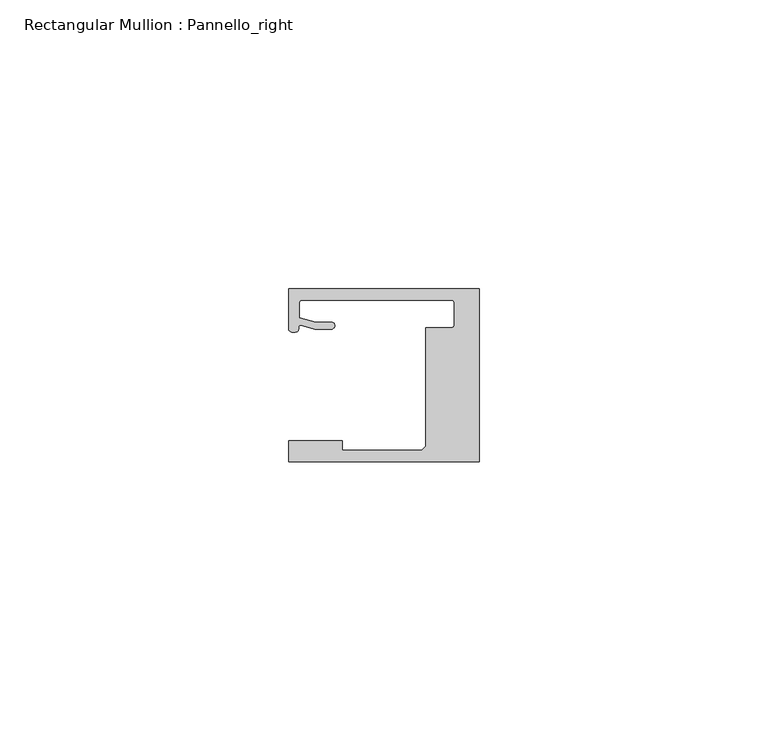
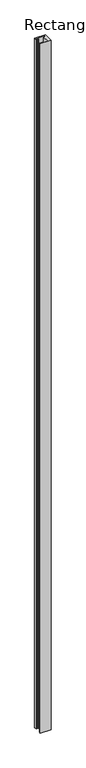
"""IFC4 building model written with IfcOpenShell, lengths in millimetres: member geometry, Rectangular Mullion : Pannello_right."""

from ifc_helpers import new_model, si_unit, frame, origin, place, context, project, spatial, polyline, circle_curve, source, transform, mapped, element, save
from ifc_brep_helpers import plane_surface, cylinder_surface, revolved_surface, extruded_surface, spline_curve, advanced_brep


def rectangular_mullion_pannello_right_08a01979(model_context):
    return source(origin(), model_context, "Body", "AdvancedBrep", [
        advanced_brep(
        [(-33.0, -15.0, 0.0), (0.0, -15.0, 0.0), (0.0, 15.0, 0.0), (-33.0000135, 15.0, 0.0), (-33.0000135, 8.0000472, 0.0), (-30.9223017, 8.6490241, 0.0), (-28.4999305, 7.9999523, 0.0), (-25.59998, 7.9999523, 0.0), (-25.59998, 9.1999523, 0.0), (-28.3419477, 9.1999523, 0.0), (-31.19998, 9.9657591, 0.0), (-31.19998, 12.50001, 0.0), (-30.69998, 13.00001, 0.0), (-4.7999726, 13.00001, 0.0), (-4.2999726, 12.50001, 0.0), (-4.2999726, 8.7500595, 0.0), (-4.7999726, 8.2500595, 0.0), (-9.2999726, 8.2500595, 0.0), (-9.2999726, -12.2999849, 0.0), (-10.0000103, -13.0000004, 0.0), (-23.700041, -13.0000004, 0.0), (-23.700041, -11.3000004, 0.0), (-33.0, -11.3000004, 0.0), (-33.0, -15.0, -2260.0), (-33.0, -11.3000004, -2260.0), (-23.700041, -11.3000004, -2260.0), (-23.700041, -13.0000004, -2260.0), (-10.0000103, -13.0000004, -2260.0), (-9.2999726, -12.2999849, -2260.0), (-9.2999726, 8.2500595, -2260.0), (-4.7999726, 8.2500595, -2260.0), (-4.2999726, 8.7500595, -2260.0), (-4.2999726, 12.50001, -2260.0), (-4.7999726, 13.00001, -2260.0), (-30.69998, 13.00001, -2260.0), (-31.19998, 12.50001, -2260.0), (-31.19998, 9.9657591, -2260.0), (-28.3419477, 9.1999523, -2260.0), (-25.59998, 9.1999523, -2260.0), (-25.59998, 7.9999523, -2260.0), (-28.4999305, 7.9999523, -2260.0), (-30.9223017, 8.6490241, -2260.0), (-33.0000135, 8.0000472, -2260.0), (-33.0000135, 15.0, -2260.0), (0.0, 15.0, -2260.0), (0.0, -15.0, -2260.0)],
        [
            (0, 1),
            (1, 2),
            (2, 3),
            (3, 4),
            (4, 5, spline_curve(3, [(-33.0000135, 8.0000472, 0.0), (-33.0000135, 7.457047519, 0.0), (-32.262327879, 7.456527435, 0.0), (-31.357433266, 7.563996614, 0.0), (-31.305645054, 7.690065204, 0.0), (-31.298563602, 8.366228555, 0.0), (-31.312054066, 8.717747958, 0.0), (-30.9223017, 8.6490241, 0.0)], [4, 2, 2, 4], [0.0, 0.0027053965905959043, 0.0058611956533709, 0.007702013405570312])),
            (5, 6),
            (6, 7),
            (7, 8, circle_curve(frame((-25.59998, 8.5999523, 0.0), z_axis=(0.0, 0.0, 1.0), x_axis=(0.0, 1.0, 0.0)), 0.6)),
            (8, 9),
            (9, 10),
            (10, 11),
            (11, 12, circle_curve(frame((-30.69998, 12.50001, 0.0), z_axis=(0.0, 0.0, -1.0), x_axis=(0.0, 1.0, 0.0)), 0.5)),
            (12, 13),
            (13, 14, circle_curve(frame((-4.7999726, 12.50001, 0.0), z_axis=(0.0, 0.0, -1.0), x_axis=(1.0, 0.0, 0.0)), 0.5)),
            (14, 15),
            (15, 16, circle_curve(frame((-4.7999726, 8.7500595, 0.0), z_axis=(0.0, 0.0, -1.0), x_axis=(0.0, -1.0, 0.0)), 0.5)),
            (16, 17),
            (17, 18),
            (18, 19),
            (19, 20),
            (20, 21),
            (21, 22),
            (22, 0),
            (23, 24),
            (24, 25),
            (25, 26),
            (26, 27),
            (27, 28),
            (28, 29),
            (29, 30),
            (30, 31, circle_curve(frame((-4.7999726, 8.7500595, -2260.0), z_axis=(0.0, 0.0, 1.0), x_axis=(0.0, -1.0, 0.0)), 0.5)),
            (31, 32),
            (32, 33, circle_curve(frame((-4.7999726, 12.50001, -2260.0), z_axis=(0.0, 0.0, 1.0), x_axis=(1.0, 0.0, 0.0)), 0.5)),
            (33, 34),
            (34, 35, circle_curve(frame((-30.69998, 12.50001, -2260.0), z_axis=(0.0, 0.0, 1.0), x_axis=(0.0, 1.0, 0.0)), 0.5)),
            (35, 36),
            (36, 37),
            (37, 38),
            (38, 39, circle_curve(frame((-25.59998, 8.5999523, -2260.0), z_axis=(0.0, 0.0, -1.0), x_axis=(0.0, 1.0, 0.0)), 0.6)),
            (39, 40),
            (40, 41),
            (41, 42, spline_curve(3, [(-30.9223017, 8.6490241, -2260.0), (-31.312054066, 8.717747958, -2260.0), (-31.298563602, 8.366228555, -2260.0), (-31.305645054, 7.690065204, -2260.0), (-31.357433266, 7.563996614, -2260.0), (-32.262327879, 7.456527435, -2260.0), (-33.0000135, 7.457047519, -2260.0), (-33.0000135, 8.0000472, -2260.0)], [4, 2, 2, 4], [0.0, 0.001840817752199412, 0.004996616814974408, 0.007702013405570312])),
            (42, 43),
            (43, 44),
            (44, 45),
            (45, 23),
            (0, 23),
            (45, 1),
            (44, 2),
            (43, 3),
            (42, 4),
            (41, 5),
            (40, 6),
            (39, 7),
            (38, 8),
            (37, 9),
            (36, 10),
            (35, 11),
            (34, 12),
            (33, 13),
            (32, 14),
            (31, 15),
            (30, 16),
            (29, 17),
            (28, 18),
            (27, 19),
            (26, 20),
            (25, 21),
            (24, 22),
        ],
        [
            plane_surface(frame((0.0, -36.2491502, 0.0), z_axis=(0.0, 0.0, 1.0), x_axis=(-1.0, 0.0, 0.0))),
            plane_surface(frame((0.0, -36.2491502, -2260.0), z_axis=(0.0, 0.0, -1.0), x_axis=(-1.0, 0.0, 0.0))),
            plane_surface(frame((-33.0, -15.0, 0.0), z_axis=(0.0, -1.0, 0.0), x_axis=(0.0, 0.0, -1.0))),
            plane_surface(frame((0.0, -15.0, 0.0), z_axis=(1.0, 0.0, 0.0), x_axis=(0.0, 0.0, -1.0))),
            plane_surface(frame((0.0, 15.0, 0.0), z_axis=(0.0, 1.0, 0.0), x_axis=(0.0, 0.0, -1.0))),
            plane_surface(frame((-33.0000135, 15.0, 0.0), z_axis=(-1.0, 0.0, 0.0), x_axis=(0.0, 0.0, -1.0))),
            extruded_surface(spline_curve(3, [(-33.0000135, 8.0000472, -2260.0), (-33.0000135, 7.457047519, -2260.0), (-32.262327879, 7.456527435, -2260.0), (-31.357433266, 7.563996614, -2260.0), (-31.305645054, 7.690065204, -2260.0), (-31.298563602, 8.366228555, -2260.0), (-31.312054066, 8.717747958, -2260.0), (-30.9223017, 8.6490241, -2260.0)], [4, 2, 2, 4], [0.0, 0.0027053965905959043, 0.0058611956533709, 0.007702013405570312]), (0.0, 0.0, 2260.0), 2260.0),
            plane_surface(frame((-30.9223017, 8.6490241, 0.0), z_axis=(-0.2588188320019168, -0.965925883389178, 0.0), x_axis=(0.0, 0.0, -1.0))),
            plane_surface(frame((-28.4999305, 7.9999523, 0.0), z_axis=(0.0, -1.0, 0.0), x_axis=(0.0, 0.0, -1.0))),
            cylinder_surface(frame((-25.59998, 8.5999523, 0.0), z_axis=(0.0, 0.0, 1.0), x_axis=(0.0, 1.0, 0.0)), 0.6),
            plane_surface(frame((-25.59998, 9.1999523, 0.0), z_axis=(0.0, 1.0, 0.0), x_axis=(0.0, 0.0, -1.0))),
            plane_surface(frame((-28.3419477, 9.1999523, 0.0), z_axis=(0.2588188320428738, 0.9659258833782035, 0.0), x_axis=(0.0, 0.0, -1.0))),
            plane_surface(frame((-31.19998, 9.9657591, 0.0), z_axis=(1.0, 0.0, 0.0), x_axis=(0.0, 0.0, -1.0))),
            revolved_surface(polyline([(-30.69998, 13.00001, -2260.0), (-30.69998, 13.00001, 0.0)]), (-30.69998, 12.50001, 0.0), (0.0, 0.0, -1.0)),
            plane_surface(frame((-30.69998, 13.00001, 0.0), z_axis=(0.0, -1.0, 0.0), x_axis=(0.0, 0.0, -1.0))),
            revolved_surface(polyline([(-4.2999726, 12.50001, -2260.0), (-4.2999726, 12.50001, 0.0)]), (-4.7999726, 12.50001, 0.0), (0.0, 0.0, -1.0)),
            plane_surface(frame((-4.2999726, 12.50001, 0.0), z_axis=(-1.0, 0.0, 0.0), x_axis=(0.0, 0.0, -1.0))),
            revolved_surface(polyline([(-4.7999726, 8.2500595, -2260.0), (-4.7999726, 8.2500595, 0.0)]), (-4.7999726, 8.7500595, 0.0), (0.0, 0.0, -1.0)),
            plane_surface(frame((-4.7999726, 8.2500595, 0.0), z_axis=(0.0, 1.0, 0.0), x_axis=(0.0, 0.0, -1.0))),
            plane_surface(frame((-9.2999726, 8.2500595, 0.0), z_axis=(-1.0, 0.0, 0.0), x_axis=(0.0, 0.0, -1.0))),
            plane_surface(frame((-9.2999726, -12.2999849, 0.0), z_axis=(-0.7070955486278075, 0.7071180135668587, 0.0), x_axis=(0.0, 0.0, -1.0))),
            plane_surface(frame((-10.0000103, -13.0000004, 0.0), z_axis=(0.0, 1.0, 0.0), x_axis=(0.0, 0.0, -1.0))),
            plane_surface(frame((-23.700041, -13.0000004, 0.0), z_axis=(1.0, 0.0, 0.0), x_axis=(0.0, 0.0, -1.0))),
            plane_surface(frame((-23.700041, -11.3000004, 0.0), z_axis=(0.0, 1.0, 0.0), x_axis=(0.0, 0.0, -1.0))),
            plane_surface(frame((-33.0, -11.3000004, 0.0), z_axis=(-1.0, 0.0, 0.0), x_axis=(0.0, 0.0, -1.0))),
        ],
        [
            (0, [[1, 2, 3, 4, 5, 6, 7, 8, 9, 10, 11, 12, 13, 14, 15, 16, 17, 18, 19, 20, 21, 22, 23]]),
            (1, [[24, 25, 26, 27, 28, 29, 30, 31, 32, 33, 34, 35, 36, 37, 38, 39, 40, 41, 42, 43, 44, 45, 46]]),
            (2, [[-1, 47, -46, 48]]),
            (3, [[-2, -48, -45, 49]]),
            (4, [[-3, -49, -44, 50]]),
            (5, [[-4, -50, -43, 51]]),
            (6, [[-5, -51, -42, 52]]),
            (7, [[-6, -52, -41, 53]]),
            (8, [[-7, -53, -40, 54]]),
            (9, [[-8, -54, -39, 55]]),
            (10, [[-9, -55, -38, 56]]),
            (11, [[-10, -56, -37, 57]]),
            (12, [[-11, -57, -36, 58]]),
            (13, [[-12, -58, -35, 59]]),
            (14, [[-13, -59, -34, 60]]),
            (15, [[-14, -60, -33, 61]]),
            (16, [[-15, -61, -32, 62]]),
            (17, [[-16, -62, -31, 63]]),
            (18, [[-17, -63, -30, 64]]),
            (19, [[-18, -64, -29, 65]]),
            (20, [[-19, -65, -28, 66]]),
            (21, [[-20, -66, -27, 67]]),
            (22, [[-21, -67, -26, 68]]),
            (23, [[-22, -68, -25, 69]]),
            (24, [[-23, -69, -24, -47]]),
        ],
    ),
    ])


if __name__ == "__main__":
    model = new_model("IFC4")
    model_context = context("Model", 3, world=origin())
    ifc_project = project(units=[si_unit("LENGTHUNIT", "METRE", prefix="MILLI")], contexts=[model_context])
    site = spatial("IfcSite", under=ifc_project)
    building = spatial("IfcBuilding", under=site)
    placement = place(None, origin())
    rectangular_mullion_pannello_right_shape = rectangular_mullion_pannello_right_08a01979(model_context)
    element("IfcMember", 1, ObjectType="Rectangular Mullion : Pannello_right", at=placement, inside=building, context=model_context, shape_type="MappedRepresentation", body=[
        mapped(rectangular_mullion_pannello_right_shape, transform((0.0, 0.0, 0.0), x_axis=(1.0, 0.0, 0.0), y_axis=(0.0, 1.0, 0.0), z_axis=(0.0, 0.0, 1.0))),
    ])
    save(model, "model.ifc")

# Revit data of these elements
# Project information
#   Project Site Name = "PROJEKTPLATS"
#   Discipline_1 = "K"
#   Discipline_2 = "I"
#   Discipline_3 = "A"
#   Discipline_4 = "M"
#   Discipline_5 = "V"
#   Project Description = "PROJEKTBESKRIVNING"
#   Project Manager = "PROJECT MANAGER"
#   Project Designer = "-"
#   Discipline_6 = "E"
#   WSP_Model_manager = "[insert name of appointed Model Manager here]"
#   WSP-K Copyright = "2019"
#   WSP Revit version = "K"
#   WSP-K Model File Path = "[insert path to Central Model here]"
#   Template = "WSP-Structure-Template-2020.rte"
#   CQSheetManagerSettings = "2|CQScale|CQHalfScale|"
#   CQPileNumberConfig = "1|PF||0|1|0|0"
#   Project Issue Date = "2018-"
#   Project Status = "Status"
#   Client Name = "BESTÄLLARE"
#   Project Address = "WSP Byggprojektering\nStreet\nZIP code City\nPhone: +4610-722 50 00\nwww.wsp.com"
#   Project Name = "PROJECT NAME"
#   Project Number = "102xxxxx"
# Type "Rectangular Mullion : Pannello_right"
#   built-in parameter 1007322 = 0.0984252 (stored number, unit not read)
#   built-in parameter 1007321 = 0.0305117 (stored number, unit not read)
#   built-in parameter 1007320 = 0 (stored number, unit not read)
